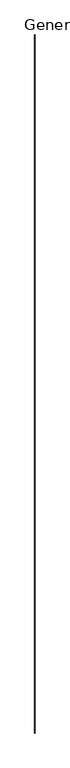
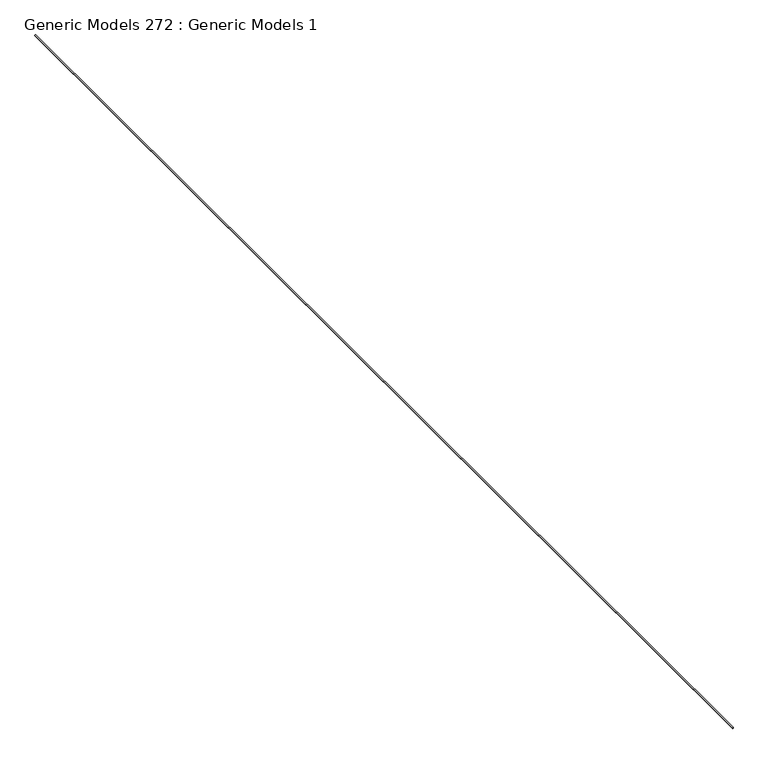
"""IFC4 building model written with IfcOpenShell, lengths in millimetres: proxy geometry, Generic Models 272 : Generic Models 1."""

import ifcopenshell
import ifcopenshell.guid

model = None  # the IFC model being written
_history = None  # IfcOwnerHistory: only IFC2X3 demands one
_inside = {}  # id of a spatial element -> (the spatial element, [elements in it])
_under = {}  # id of a project, library or spatial element -> (it, [spatial elements below it])
_declared = {}  # id of a project -> (the project, [libraries it declares])
_typed = {}  # id of a type object -> (the type object, [elements of that type])
_made_of = {}  # id of a material, layer set ... -> (it, [elements and type objects made of it])


def new_model(schema):
    """Start an empty IFC model of exactly this schema.

    Asked for "IFC4X3", IfcOpenShell would pick the latest addendum, in which some entities
    have other attributes; the version numbers below select the first issue.
    IFC2X3 requires an IfcOwnerHistory on every rooted entity: one is made here for all.
    """
    global model, _history
    if schema == "IFC4X3":
        model = ifcopenshell.file(schema_version=(4, 3, 0, 0))
    else:
        model = ifcopenshell.file(schema=schema)
    _inside.clear()
    _under.clear()
    _declared.clear()
    _typed.clear()
    _made_of.clear()
    _history = None
    if model.schema == "IFC2X3":
        org = make("IfcOrganization", Name="unknown")
        user = make(
            "IfcPersonAndOrganization",
            ThePerson=make("IfcPerson", FamilyName="unknown"),
            TheOrganization=org,
        )
        app = make(
            "IfcApplication",
            ApplicationDeveloper=org,
            Version="unknown",
            ApplicationFullName="unknown",
            ApplicationIdentifier="unknown",
        )
        _history = make(
            "IfcOwnerHistory",
            OwningUser=user,
            OwningApplication=app,
            ChangeAction="ADDED",
            CreationDate=0,
        )
    return model


def make(cls, **values):
    """One entity of the class cls with the attributes given. An attribute that is None is left unset."""
    return model.create_entity(
        cls, **{name: value for name, value in values.items() if value is not None}
    )


def rooted(cls, **values):
    """An entity with a GlobalId (a new one), such as an element, a storey or a relation."""
    return make(cls, GlobalId=ifcopenshell.guid.new(), OwnerHistory=_history, **values)


def si_unit(unit_type, name, prefix=None):
    """IfcSIUnit, for example si_unit("LENGTHUNIT", "METRE", prefix="MILLI")."""
    return make("IfcSIUnit", UnitType=unit_type, Prefix=prefix, Name=name)


def assignment(units):
    """IfcUnitAssignment: the units of a project."""
    return None if units is None else make("IfcUnitAssignment", Units=units)


def point(xyz):
    """IfcCartesianPoint."""
    return None if xyz is None else make("IfcCartesianPoint", Coordinates=xyz)


def direction(xyz):
    """IfcDirection."""
    return None if xyz is None else make("IfcDirection", DirectionRatios=xyz)


def frame(location, z_axis=None, x_axis=None):
    """IfcAxis2Placement3D, a coordinate frame: its origin and axes. An axis left out is left unset."""
    return make(
        "IfcAxis2Placement3D",
        Location=point(location),
        Axis=direction(z_axis),
        RefDirection=direction(x_axis),
    )


def frame_2d(location, x_axis=None):
    """IfcAxis2Placement2D, a coordinate frame in the plane: its origin and x axis."""
    return make(
        "IfcAxis2Placement2D", Location=point(location), RefDirection=direction(x_axis)
    )


def origin():
    """The frame at (0, 0, 0) with its axes left unset."""
    return frame((0.0, 0.0, 0.0))


def place(relative_to, where):
    """IfcLocalPlacement: puts the frame where relative to a parent placement (None: the world)."""
    return make(
        "IfcLocalPlacement", PlacementRelTo=relative_to, RelativePlacement=where
    )


def context(
    kind, dimensions, precision=None, world=None, true_north=None, identifier=None
):
    """IfcGeometricRepresentationContext, for example the 3D "Model" context."""
    return make(
        "IfcGeometricRepresentationContext",
        ContextIdentifier=identifier,
        ContextType=kind,
        CoordinateSpaceDimension=dimensions,
        Precision=precision,
        WorldCoordinateSystem=world,
        TrueNorth=true_north,
    )


def project(units=None, contexts=None):
    """IfcProject with its units and contexts."""
    return rooted(
        "IfcProject",
        Name="project",
        RepresentationContexts=contexts,
        UnitsInContext=assignment(units),
    )


def spatial(cls, under=None, at=None, **own):
    """A site, building, storey or space (cls), placed at a placement, below another one or the project."""
    s = rooted(cls, ObjectPlacement=at, **own)
    if under is not None:
        _under.setdefault(under.id(), (under, []))[1].append(s)
    return s


def polyline(points):
    """IfcPolyline through the points."""
    return make("IfcPolyline", Points=[point(p) for p in points])


def circle_curve(where, radius):
    """IfcCircle in the frame where."""
    return make("IfcCircle", Position=where, Radius=radius)


def trimmed(basis, trim1, trim2, sense, master):
    """IfcTrimmedCurve: the piece of a basis curve between two trims."""
    return make(
        "IfcTrimmedCurve",
        BasisCurve=basis,
        Trim1=trim1,
        Trim2=trim2,
        SenseAgreement=sense,
        MasterRepresentation=master,
    )


def segment(curve, same_sense, transition):
    """IfcCompositeCurveSegment."""
    return make(
        "IfcCompositeCurveSegment",
        Transition=transition,
        SameSense=same_sense,
        ParentCurve=curve,
    )


def composite_curve(segments, self_intersect=None):
    """IfcCompositeCurve: segments joined end to end."""
    return make("IfcCompositeCurve", Segments=segments, SelfIntersect=self_intersect)


def outline(outer, holes=None, kind="AREA"):
    """IfcArbitraryClosedProfileDef: a profile drawn as a closed curve; with holes, ...WithVoids."""
    if holes is None:
        return make("IfcArbitraryClosedProfileDef", ProfileType=kind, OuterCurve=outer)
    return make(
        "IfcArbitraryProfileDefWithVoids",
        ProfileType=kind,
        OuterCurve=outer,
        InnerCurves=holes,
    )


def extrude(swept, where, along, depth):
    """IfcExtrudedAreaSolid: the profile swept, set in the frame where, extruded along a direction by depth."""
    return make(
        "IfcExtrudedAreaSolid",
        SweptArea=swept,
        Position=where,
        ExtrudedDirection=direction(along),
        Depth=depth,
    )


def shape(context_of_items, identifier, shape_type, items):
    """IfcShapeRepresentation: the items that make up one representation, for example the "Body"."""
    return make(
        "IfcShapeRepresentation",
        ContextOfItems=context_of_items,
        RepresentationIdentifier=identifier,
        RepresentationType=shape_type,
        Items=items,
    )


def source(mapping_origin, context_of_items, identifier, shape_type, items):
    """IfcRepresentationMap: a shape defined once, which mapped items show again and again."""
    return make(
        "IfcRepresentationMap",
        MappingOrigin=mapping_origin,
        MappedRepresentation=shape(context_of_items, identifier, shape_type, items),
    )


def transform(
    local_origin,
    x_axis=None,
    y_axis=None,
    z_axis=None,
    scale=None,
    scale2=None,
    scale3=None,
    uniform=True,
):
    """IfcCartesianTransformationOperator3D, or its non-uniform kind. x_axis, y_axis, z_axis: its Axis1, 2, 3."""
    if uniform:
        return make(
            "IfcCartesianTransformationOperator3D",
            Axis1=direction(x_axis),
            Axis2=direction(y_axis),
            LocalOrigin=point(local_origin),
            Scale=scale,
            Axis3=direction(z_axis),
        )
    return make(
        "IfcCartesianTransformationOperator3DnonUniform",
        Axis1=direction(x_axis),
        Axis2=direction(y_axis),
        LocalOrigin=point(local_origin),
        Scale=scale,
        Axis3=direction(z_axis),
        Scale2=scale2,
        Scale3=scale3,
    )


def mapped(mapping_source, mapping_target):
    """IfcMappedItem: shows the shape of a source again, moved by a transform."""
    return make(
        "IfcMappedItem", MappingSource=mapping_source, MappingTarget=mapping_target
    )


def made_of(thing, what):
    """Note that an element or type object is made of a material, layer set ...; save() writes the relation."""
    if what is not None:
        _made_of.setdefault(what.id(), (what, []))[1].append(thing)
    return thing


def element(
    cls,
    number,
    at=None,
    inside=None,
    cuts=None,
    type_object=None,
    material=None,
    context=None,
    identifier="Body",
    shape_type=None,
    held_by="IfcProductDefinitionShape",
    body=None,
    shapes=None,
    **own,
):
    """One element of the class cls, such as IfcWall. Its Tag is "e" and its number.

    at: its placement. inside: the storey or other place that contains it. cuts: it is an
    opening in that element (IfcRelVoidsElement). A single representation is given by context,
    identifier, shape_type and body (its items); several are given by shapes. held_by: the class
    of the entity that holds the representations. save() writes the other relations.
    """
    e = rooted(cls, Tag="e%d" % number, ObjectPlacement=at, **own)
    if body is not None:
        shapes = [shape(context, identifier, shape_type, body)]
    if shapes is not None:
        e.Representation = make(held_by, Representations=shapes)
    if inside is not None:
        _inside.setdefault(inside.id(), (inside, []))[1].append(e)
    if cuts is not None:
        rooted(
            "IfcRelVoidsElement", RelatingBuildingElement=cuts, RelatedOpeningElement=e
        )
    if type_object is not None:
        _typed.setdefault(type_object.id(), (type_object, []))[1].append(e)
    return made_of(e, material)


def aggregate(whole, parts):
    """IfcRelAggregates: a whole, such as a stair, and the parts it consists of."""
    return rooted("IfcRelAggregates", RelatingObject=whole, RelatedObjects=parts)


def save(model, path):
    """Write the relations noted so far, then the file.

    IfcRelAggregates (storeys below a building ...), IfcRelContainedInSpatialStructure (elements
    in a storey), IfcRelDefinesByType, IfcRelAssociatesMaterial and IfcRelDeclares: one each for
    every whole, place, type object, material and project.
    """
    for whole, parts in _under.values():
        aggregate(whole, parts)
    for where, things in _inside.values():
        rooted(
            "IfcRelContainedInSpatialStructure",
            RelatedElements=things,
            RelatingStructure=where,
        )
    for kind, things in _typed.values():
        rooted("IfcRelDefinesByType", RelatedObjects=things, RelatingType=kind)
    for what, things in _made_of.values():
        rooted("IfcRelAssociatesMaterial", RelatedObjects=things, RelatingMaterial=what)
    for by, libraries in _declared.values():
        rooted("IfcRelDeclares", RelatingContext=by, RelatedDefinitions=libraries)
    model.write(path)


def generic_models_272_generic_models_1_04ec0b07(model_context):
    return source(origin(), model_context, "Body", "SweptSolid", [
        extrude(outline(composite_curve([segment(polyline([(123440.571, 1521.9214201), (123450.096, 1521.9214201)]), True, "CONTINUOUS"), segment(trimmed(circle_curve(frame_2d((123453.0107405, 1518.7464201)), 4.3100275), [point((123450.096, 1521.9214201))], [point((123450.096, 1515.5714201))], True, "CARTESIAN"), True, "CONTINUOUS"), segment(polyline([(123450.096, 1515.5714201), (123440.571, 1515.5714201)]), True, "CONTINUOUS"), segment(trimmed(circle_curve(frame_2d((123443.4857405, 1518.7464201)), 4.3100275), [point((123440.571, 1515.5714201))], [point((123440.571, 1521.9214201))], False, "CARTESIAN"), True, "CONTINUOUS")], self_intersect=False)), frame((0.0, -5493.3230338, 0.0), z_axis=(0.0, 1.0, 0.0), x_axis=(0.0, 0.0, 1.0)), (0.0, 0.0, 1.0), 12344.4),
    ])


if __name__ == "__main__":
    model = new_model("IFC4")
    model_context = context("Model", 3, world=origin())
    ifc_project = project(units=[si_unit("LENGTHUNIT", "METRE", prefix="MILLI")], contexts=[model_context])
    site = spatial("IfcSite", under=ifc_project)
    building = spatial("IfcBuilding", under=site)
    placement = place(None, origin())
    generic_models_272_generic_models_1_shape = generic_models_272_generic_models_1_04ec0b07(model_context)
    element("IfcBuildingElementProxy", 1, Name="Generic Models 272 : Generic Models 1", ObjectType="Generic Models 272 : Generic Models 1", at=placement, inside=building, context=model_context, shape_type="MappedRepresentation", body=[
        mapped(generic_models_272_generic_models_1_shape, transform((0.0, 0.0, 0.0), x_axis=(1.0, 0.0, 0.0), y_axis=(0.0, 1.0, 0.0), z_axis=(0.0, 0.0, 1.0))),
    ])
    save(model, "model.ifc")

# Revit data of these elements
# Element 1 (IfcBuildingElementProxy, "Generic Models 272 : Generic Models 1")
#   Materials on its faces: "_SEALANT JOINT"
# Materials
#   "_SEALANT JOINT": class "Generic", colour RGB 190 220 196, transparency 0, Cost = 0
